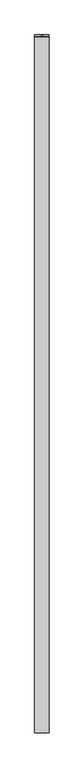
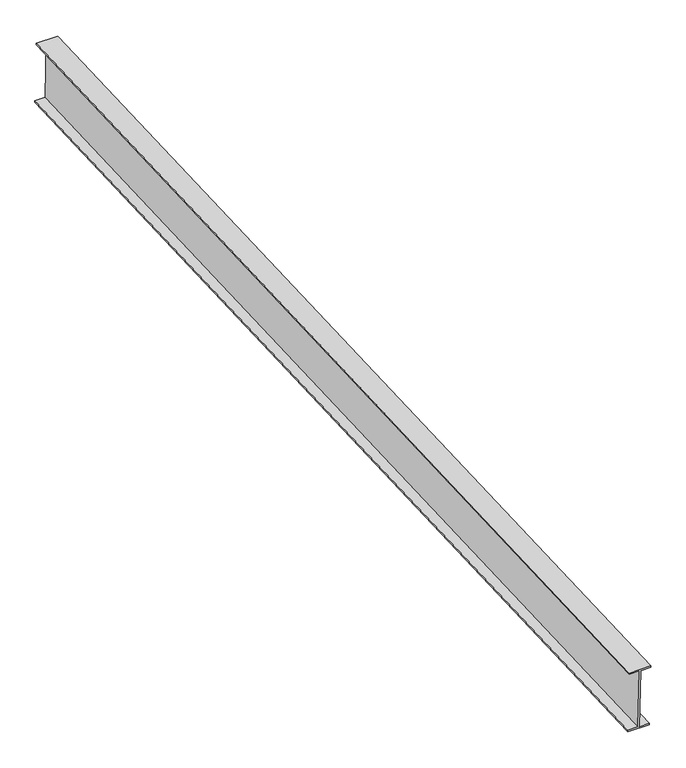
"""IFC4 building model written with IfcOpenShell, lengths in millimetres: proxy geometry, Generic Models 7:Generic Models 1:1:Generic Models 1:1 : Generic Models 7:Generic Models 1:337419:21 : Generic Models 7:Generic Models 1:1:Generic Models 1:1 : Generic Models 7:Generic Models 1:337419:306201."""

import ifcopenshell
import ifcopenshell.guid

model = None  # the IFC model being written
_history = None  # IfcOwnerHistory: only IFC2X3 demands one
_inside = {}  # id of a spatial element -> (the spatial element, [elements in it])
_under = {}  # id of a project, library or spatial element -> (it, [spatial elements below it])
_declared = {}  # id of a project -> (the project, [libraries it declares])
_typed = {}  # id of a type object -> (the type object, [elements of that type])
_made_of = {}  # id of a material, layer set ... -> (it, [elements and type objects made of it])


def new_model(schema):
    """Start an empty IFC model of exactly this schema.

    Asked for "IFC4X3", IfcOpenShell would pick the latest addendum, in which some entities
    have other attributes; the version numbers below select the first issue.
    IFC2X3 requires an IfcOwnerHistory on every rooted entity: one is made here for all.
    """
    global model, _history
    if schema == "IFC4X3":
        model = ifcopenshell.file(schema_version=(4, 3, 0, 0))
    else:
        model = ifcopenshell.file(schema=schema)
    _inside.clear()
    _under.clear()
    _declared.clear()
    _typed.clear()
    _made_of.clear()
    _history = None
    if model.schema == "IFC2X3":
        org = make("IfcOrganization", Name="unknown")
        user = make(
            "IfcPersonAndOrganization",
            ThePerson=make("IfcPerson", FamilyName="unknown"),
            TheOrganization=org,
        )
        app = make(
            "IfcApplication",
            ApplicationDeveloper=org,
            Version="unknown",
            ApplicationFullName="unknown",
            ApplicationIdentifier="unknown",
        )
        _history = make(
            "IfcOwnerHistory",
            OwningUser=user,
            OwningApplication=app,
            ChangeAction="ADDED",
            CreationDate=0,
        )
    return model


def make(cls, **values):
    """One entity of the class cls with the attributes given. An attribute that is None is left unset."""
    return model.create_entity(
        cls, **{name: value for name, value in values.items() if value is not None}
    )


def rooted(cls, **values):
    """An entity with a GlobalId (a new one), such as an element, a storey or a relation."""
    return make(cls, GlobalId=ifcopenshell.guid.new(), OwnerHistory=_history, **values)


def si_unit(unit_type, name, prefix=None):
    """IfcSIUnit, for example si_unit("LENGTHUNIT", "METRE", prefix="MILLI")."""
    return make("IfcSIUnit", UnitType=unit_type, Prefix=prefix, Name=name)


def assignment(units):
    """IfcUnitAssignment: the units of a project."""
    return None if units is None else make("IfcUnitAssignment", Units=units)


def point(xyz):
    """IfcCartesianPoint."""
    return None if xyz is None else make("IfcCartesianPoint", Coordinates=xyz)


def direction(xyz):
    """IfcDirection."""
    return None if xyz is None else make("IfcDirection", DirectionRatios=xyz)


def frame(location, z_axis=None, x_axis=None):
    """IfcAxis2Placement3D, a coordinate frame: its origin and axes. An axis left out is left unset."""
    return make(
        "IfcAxis2Placement3D",
        Location=point(location),
        Axis=direction(z_axis),
        RefDirection=direction(x_axis),
    )


def origin():
    """The frame at (0, 0, 0) with its axes left unset."""
    return frame((0.0, 0.0, 0.0))


def place(relative_to, where):
    """IfcLocalPlacement: puts the frame where relative to a parent placement (None: the world)."""
    return make(
        "IfcLocalPlacement", PlacementRelTo=relative_to, RelativePlacement=where
    )


def context(
    kind, dimensions, precision=None, world=None, true_north=None, identifier=None
):
    """IfcGeometricRepresentationContext, for example the 3D "Model" context."""
    return make(
        "IfcGeometricRepresentationContext",
        ContextIdentifier=identifier,
        ContextType=kind,
        CoordinateSpaceDimension=dimensions,
        Precision=precision,
        WorldCoordinateSystem=world,
        TrueNorth=true_north,
    )


def project(units=None, contexts=None):
    """IfcProject with its units and contexts."""
    return rooted(
        "IfcProject",
        Name="project",
        RepresentationContexts=contexts,
        UnitsInContext=assignment(units),
    )


def spatial(cls, under=None, at=None, **own):
    """A site, building, storey or space (cls), placed at a placement, below another one or the project."""
    s = rooted(cls, ObjectPlacement=at, **own)
    if under is not None:
        _under.setdefault(under.id(), (under, []))[1].append(s)
    return s


def polyline(points):
    """IfcPolyline through the points."""
    return make("IfcPolyline", Points=[point(p) for p in points])


def outline(outer, holes=None, kind="AREA"):
    """IfcArbitraryClosedProfileDef: a profile drawn as a closed curve; with holes, ...WithVoids."""
    if holes is None:
        return make("IfcArbitraryClosedProfileDef", ProfileType=kind, OuterCurve=outer)
    return make(
        "IfcArbitraryProfileDefWithVoids",
        ProfileType=kind,
        OuterCurve=outer,
        InnerCurves=holes,
    )


def extrude(swept, where, along, depth):
    """IfcExtrudedAreaSolid: the profile swept, set in the frame where, extruded along a direction by depth."""
    return make(
        "IfcExtrudedAreaSolid",
        SweptArea=swept,
        Position=where,
        ExtrudedDirection=direction(along),
        Depth=depth,
    )


def shape(context_of_items, identifier, shape_type, items):
    """IfcShapeRepresentation: the items that make up one representation, for example the "Body"."""
    return make(
        "IfcShapeRepresentation",
        ContextOfItems=context_of_items,
        RepresentationIdentifier=identifier,
        RepresentationType=shape_type,
        Items=items,
    )


def source(mapping_origin, context_of_items, identifier, shape_type, items):
    """IfcRepresentationMap: a shape defined once, which mapped items show again and again."""
    return make(
        "IfcRepresentationMap",
        MappingOrigin=mapping_origin,
        MappedRepresentation=shape(context_of_items, identifier, shape_type, items),
    )


def transform(
    local_origin,
    x_axis=None,
    y_axis=None,
    z_axis=None,
    scale=None,
    scale2=None,
    scale3=None,
    uniform=True,
):
    """IfcCartesianTransformationOperator3D, or its non-uniform kind. x_axis, y_axis, z_axis: its Axis1, 2, 3."""
    if uniform:
        return make(
            "IfcCartesianTransformationOperator3D",
            Axis1=direction(x_axis),
            Axis2=direction(y_axis),
            LocalOrigin=point(local_origin),
            Scale=scale,
            Axis3=direction(z_axis),
        )
    return make(
        "IfcCartesianTransformationOperator3DnonUniform",
        Axis1=direction(x_axis),
        Axis2=direction(y_axis),
        LocalOrigin=point(local_origin),
        Scale=scale,
        Axis3=direction(z_axis),
        Scale2=scale2,
        Scale3=scale3,
    )


def mapped(mapping_source, mapping_target):
    """IfcMappedItem: shows the shape of a source again, moved by a transform."""
    return make(
        "IfcMappedItem", MappingSource=mapping_source, MappingTarget=mapping_target
    )


def made_of(thing, what):
    """Note that an element or type object is made of a material, layer set ...; save() writes the relation."""
    if what is not None:
        _made_of.setdefault(what.id(), (what, []))[1].append(thing)
    return thing


def element(
    cls,
    number,
    at=None,
    inside=None,
    cuts=None,
    type_object=None,
    material=None,
    context=None,
    identifier="Body",
    shape_type=None,
    held_by="IfcProductDefinitionShape",
    body=None,
    shapes=None,
    **own,
):
    """One element of the class cls, such as IfcWall. Its Tag is "e" and its number.

    at: its placement. inside: the storey or other place that contains it. cuts: it is an
    opening in that element (IfcRelVoidsElement). A single representation is given by context,
    identifier, shape_type and body (its items); several are given by shapes. held_by: the class
    of the entity that holds the representations. save() writes the other relations.
    """
    e = rooted(cls, Tag="e%d" % number, ObjectPlacement=at, **own)
    if body is not None:
        shapes = [shape(context, identifier, shape_type, body)]
    if shapes is not None:
        e.Representation = make(held_by, Representations=shapes)
    if inside is not None:
        _inside.setdefault(inside.id(), (inside, []))[1].append(e)
    if cuts is not None:
        rooted(
            "IfcRelVoidsElement", RelatingBuildingElement=cuts, RelatedOpeningElement=e
        )
    if type_object is not None:
        _typed.setdefault(type_object.id(), (type_object, []))[1].append(e)
    return made_of(e, material)


def aggregate(whole, parts):
    """IfcRelAggregates: a whole, such as a stair, and the parts it consists of."""
    return rooted("IfcRelAggregates", RelatingObject=whole, RelatedObjects=parts)


def save(model, path):
    """Write the relations noted so far, then the file.

    IfcRelAggregates (storeys below a building ...), IfcRelContainedInSpatialStructure (elements
    in a storey), IfcRelDefinesByType, IfcRelAssociatesMaterial and IfcRelDeclares: one each for
    every whole, place, type object, material and project.
    """
    for whole, parts in _under.values():
        aggregate(whole, parts)
    for where, things in _inside.values():
        rooted(
            "IfcRelContainedInSpatialStructure",
            RelatedElements=things,
            RelatingStructure=where,
        )
    for kind, things in _typed.values():
        rooted("IfcRelDefinesByType", RelatedObjects=things, RelatingType=kind)
    for what, things in _made_of.values():
        rooted("IfcRelAssociatesMaterial", RelatedObjects=things, RelatingMaterial=what)
    for by, libraries in _declared.values():
        rooted("IfcRelDeclares", RelatingContext=by, RelatedDefinitions=libraries)
    model.write(path)


def generic_models_3e432a6c(model_context):
    return source(origin(), model_context, "Body", "SweptSolid", [
        extrude(outline(polyline([(126.873, 0.0), (126.873, -6.3500001), (78.994, -6.3500001), (78.994, -295.0294372), (126.873, -295.0294372), (126.873, -301.3794372), (25.527, -301.3794372), (25.527, -295.0294372), (73.406, -295.0294372), (73.406, -6.3500001), (25.527, -6.3500001), (25.527, 0.0), (126.873, 0.0)])), frame((579256.911724, -578815.1475699, 3695.4094554), z_axis=(0.0, 0.9991330730920968, 0.041630544718308224), x_axis=(-1.0, 0.0, 0.0)), (0.0, 0.0, 1.0), 4876.8),
    ])


if __name__ == "__main__":
    model = new_model("IFC4")
    model_context = context("Model", 3, world=origin())
    ifc_project = project(units=[si_unit("LENGTHUNIT", "METRE", prefix="MILLI")], contexts=[model_context])
    site = spatial("IfcSite", under=ifc_project)
    building = spatial("IfcBuilding", under=site)
    placement = place(None, origin())
    generic_models_shape = generic_models_3e432a6c(model_context)
    element("IfcBuildingElementProxy", 1, Name="Generic Models 7:Generic Models 1:1:Generic Models 1:1 : Generic Models 7:Generic Models 1:337419:21 : Generic Models 7:Generic Models 1:1:Generic Models 1:1 : Generic Models 7:Generic Models 1:337419:306201", ObjectType="Generic Models 7:Generic Models 1:1:Generic Models 1:1 : Generic Models 7:Generic Models 1:337419:21 : Generic Models 7:Generic Models 1:1:Generic Models 1:1 : Generic Models 7:Generic Models 1:337419:306201", at=placement, inside=building, context=model_context, shape_type="MappedRepresentation", body=[
        mapped(generic_models_shape, transform((0.0, 0.0, 0.0), x_axis=(1.0, 0.0, 0.0), y_axis=(0.0, 1.0, 0.0), z_axis=(0.0, 0.0, 1.0))),
    ])
    save(model, "model.ifc")

# Revit data of these elements
# Type "Generic Models 7:Generic Models 1:1:Generic Models 1:1 : Generic Models 7:Generic Models 1:337419:21 : Generic Models 7:Generic Models 1:1:Generic Models 1:1 : Generic Models 7:Generic Models 1:337419:306201"
#   NameOverride = "Generic Models 7:Generic Models 1:1:Generic Models 1:1 : Generic Models 7:Generic Models 1:337419:306201"
#   ObjectTypeOverride = "Generic Models 1:1 : Generic Models 7:Generic Models 1:337419"
#   Reference = "Generic Models 1"
#   Tag = "306201"
# Element 1 (IfcBuildingElementProxy, "Generic Models 7:Generic Models 1:1:Generic Models 1:1 : Generic Models 7:Generic Models 1:337419:21 : Generic Models 7:Generic Models 1:1:Generic Models 1:1 : Generic Models 7:Generic Models 1:337419:306201")
#   Materials on its faces: "'ZEE' SECTION (8.0x3.5Z - SEE STRUCT. DWGS)"
# Materials
#   "'ZEE' SECTION (8.0x3.5Z - SEE STRUCT. DWGS)": class "Unassigned", colour RGB 210 209 208, transparency 0, Keynote = "M05121300.02", Cost = 0
